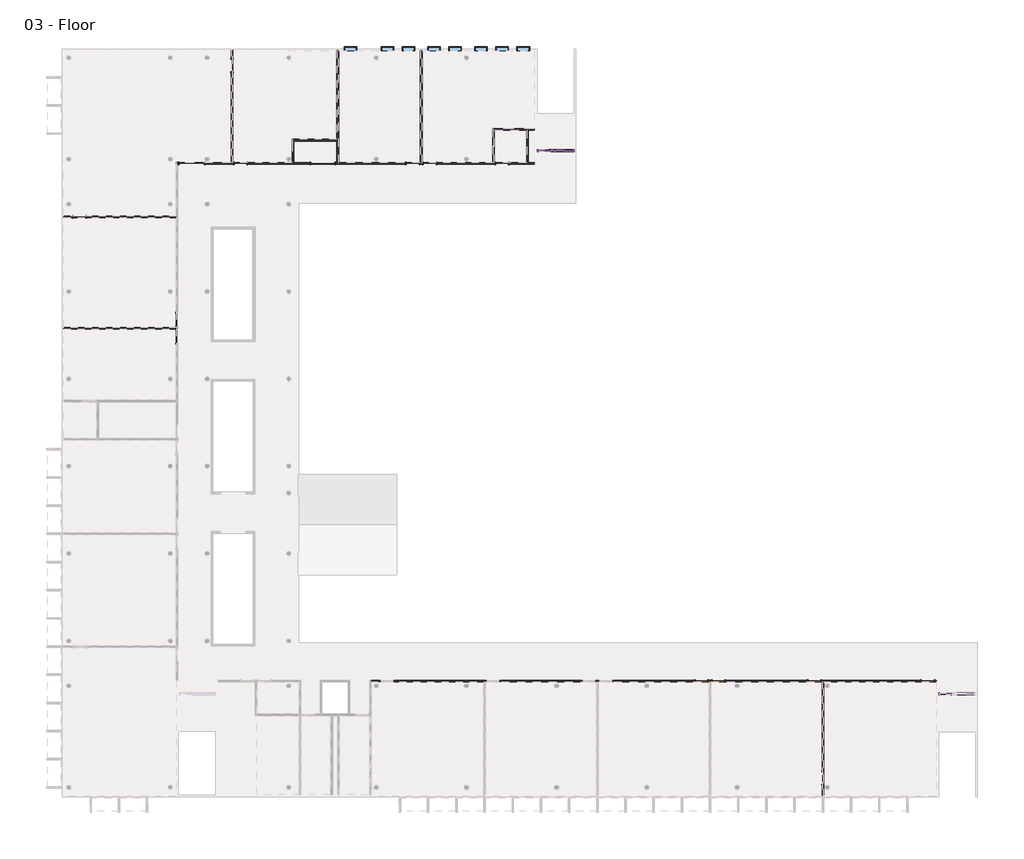
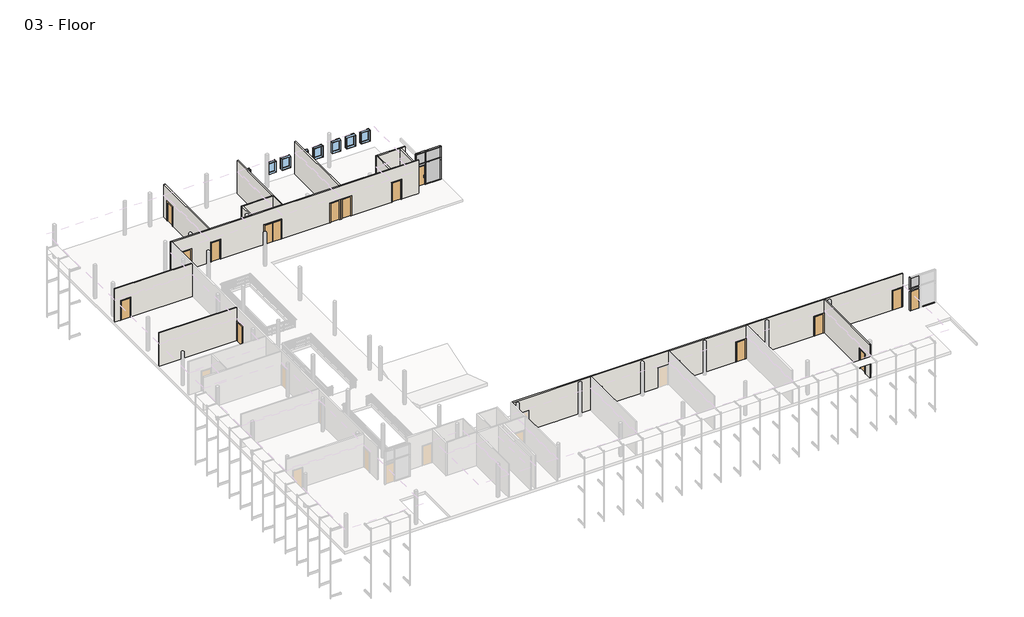
# One storey, part 2 of 4: 22 members, 17 doors, 13 walls, 8 windows, 6 plates.
"""IFC4 building model written with IfcOpenShell, lengths in millimetres."""

import ifcopenshell
import ifcopenshell.guid

model = None  # the IFC model being written
_history = None  # IfcOwnerHistory: only IFC2X3 demands one
_inside = {}  # id of a spatial element -> (the spatial element, [elements in it])
_under = {}  # id of a project, library or spatial element -> (it, [spatial elements below it])
_declared = {}  # id of a project -> (the project, [libraries it declares])
_typed = {}  # id of a type object -> (the type object, [elements of that type])
_made_of = {}  # id of a material, layer set ... -> (it, [elements and type objects made of it])


def new_model(schema):
    """Start an empty IFC model of exactly this schema.

    Asked for "IFC4X3", IfcOpenShell would pick the latest addendum, in which some entities
    have other attributes; the version numbers below select the first issue.
    IFC2X3 requires an IfcOwnerHistory on every rooted entity: one is made here for all.
    """
    global model, _history
    if schema == "IFC4X3":
        model = ifcopenshell.file(schema_version=(4, 3, 0, 0))
    else:
        model = ifcopenshell.file(schema=schema)
    _inside.clear()
    _under.clear()
    _declared.clear()
    _typed.clear()
    _made_of.clear()
    _history = None
    if model.schema == "IFC2X3":
        org = make("IfcOrganization", Name="unknown")
        user = make(
            "IfcPersonAndOrganization",
            ThePerson=make("IfcPerson", FamilyName="unknown"),
            TheOrganization=org,
        )
        app = make(
            "IfcApplication",
            ApplicationDeveloper=org,
            Version="unknown",
            ApplicationFullName="unknown",
            ApplicationIdentifier="unknown",
        )
        _history = make(
            "IfcOwnerHistory",
            OwningUser=user,
            OwningApplication=app,
            ChangeAction="ADDED",
            CreationDate=0,
        )
    return model


def make(cls, **values):
    """One entity of the class cls with the attributes given. An attribute that is None is left unset."""
    return model.create_entity(
        cls, **{name: value for name, value in values.items() if value is not None}
    )


def rooted(cls, **values):
    """An entity with a GlobalId (a new one), such as an element, a storey or a relation."""
    return make(cls, GlobalId=ifcopenshell.guid.new(), OwnerHistory=_history, **values)


def si_unit(unit_type, name, prefix=None):
    """IfcSIUnit, for example si_unit("LENGTHUNIT", "METRE", prefix="MILLI")."""
    return make("IfcSIUnit", UnitType=unit_type, Prefix=prefix, Name=name)


def assignment(units):
    """IfcUnitAssignment: the units of a project."""
    return None if units is None else make("IfcUnitAssignment", Units=units)


def point(xyz):
    """IfcCartesianPoint."""
    return None if xyz is None else make("IfcCartesianPoint", Coordinates=xyz)


def direction(xyz):
    """IfcDirection."""
    return None if xyz is None else make("IfcDirection", DirectionRatios=xyz)


def frame(location, z_axis=None, x_axis=None):
    """IfcAxis2Placement3D, a coordinate frame: its origin and axes. An axis left out is left unset."""
    return make(
        "IfcAxis2Placement3D",
        Location=point(location),
        Axis=direction(z_axis),
        RefDirection=direction(x_axis),
    )


def origin():
    """The frame at (0, 0, 0) with its axes left unset."""
    return frame((0.0, 0.0, 0.0))


def origin_with_axes():
    """The frame at (0, 0, 0) with the z axis (0, 0, 1) and the x axis (1, 0, 0) written out."""
    return frame((0.0, 0.0, 0.0), z_axis=(0.0, 0.0, 1.0), x_axis=(1.0, 0.0, 0.0))


def place(relative_to, where):
    """IfcLocalPlacement: puts the frame where relative to a parent placement (None: the world)."""
    return make(
        "IfcLocalPlacement", PlacementRelTo=relative_to, RelativePlacement=where
    )


def context(
    kind, dimensions, precision=None, world=None, true_north=None, identifier=None
):
    """IfcGeometricRepresentationContext, for example the 3D "Model" context."""
    return make(
        "IfcGeometricRepresentationContext",
        ContextIdentifier=identifier,
        ContextType=kind,
        CoordinateSpaceDimension=dimensions,
        Precision=precision,
        WorldCoordinateSystem=world,
        TrueNorth=true_north,
    )


def project(units=None, contexts=None):
    """IfcProject with its units and contexts."""
    return rooted(
        "IfcProject",
        Name="project",
        RepresentationContexts=contexts,
        UnitsInContext=assignment(units),
    )


def spatial(cls, under=None, at=None, **own):
    """A site, building, storey or space (cls), placed at a placement, below another one or the project."""
    s = rooted(cls, ObjectPlacement=at, **own)
    if under is not None:
        _under.setdefault(under.id(), (under, []))[1].append(s)
    return s


def polyline(points):
    """IfcPolyline through the points."""
    return make("IfcPolyline", Points=[point(p) for p in points])


def outline(outer, holes=None, kind="AREA"):
    """IfcArbitraryClosedProfileDef: a profile drawn as a closed curve; with holes, ...WithVoids."""
    if holes is None:
        return make("IfcArbitraryClosedProfileDef", ProfileType=kind, OuterCurve=outer)
    return make(
        "IfcArbitraryProfileDefWithVoids",
        ProfileType=kind,
        OuterCurve=outer,
        InnerCurves=holes,
    )


def extrude(swept, where, along, depth):
    """IfcExtrudedAreaSolid: the profile swept, set in the frame where, extruded along a direction by depth."""
    return make(
        "IfcExtrudedAreaSolid",
        SweptArea=swept,
        Position=where,
        ExtrudedDirection=direction(along),
        Depth=depth,
    )


def faces_of(points, faces, orient=None, outer=None):
    """IfcFace entities. A face is a list of loops; a loop is a list of indices into points, from 0.

    orient and outer hold one flag for each loop. By default every Orientation is true, the
    first loop of a face is its IfcFaceOuterBound and the others are IfcFaceBound.
    """
    made = []
    for i, loops in enumerate(faces):
        bounds = []
        for j, loop in enumerate(loops):
            is_outer = j == 0 if outer is None else outer[i][j]
            bounds.append(
                make(
                    "IfcFaceOuterBound" if is_outer else "IfcFaceBound",
                    Bound=make("IfcPolyLoop", Polygon=[points[k] for k in loop]),
                    Orientation=True if orient is None else orient[i][j],
                )
            )
        made.append(make("IfcFace", Bounds=bounds))
    return made


def faceted_brep(points, faces, orient=None, outer=None, voids=None):
    """IfcFacetedBrep: a solid bounded by flat faces; with voids (closed shells), ...WithVoids."""
    shared = [point(p) for p in points]
    hull = make("IfcClosedShell", CfsFaces=faces_of(shared, faces, orient, outer))
    if voids is None:
        return make("IfcFacetedBrep", Outer=hull)
    return make(
        "IfcFacetedBrepWithVoids",
        Outer=hull,
        Voids=[
            make(cls, CfsFaces=faces_of(shared, fs, o, b)) for cls, fs, o, b in voids
        ],
    )


def shape(context_of_items, identifier, shape_type, items):
    """IfcShapeRepresentation: the items that make up one representation, for example the "Body"."""
    return make(
        "IfcShapeRepresentation",
        ContextOfItems=context_of_items,
        RepresentationIdentifier=identifier,
        RepresentationType=shape_type,
        Items=items,
    )


def source(mapping_origin, context_of_items, identifier, shape_type, items):
    """IfcRepresentationMap: a shape defined once, which mapped items show again and again."""
    return make(
        "IfcRepresentationMap",
        MappingOrigin=mapping_origin,
        MappedRepresentation=shape(context_of_items, identifier, shape_type, items),
    )


def transform(
    local_origin,
    x_axis=None,
    y_axis=None,
    z_axis=None,
    scale=None,
    scale2=None,
    scale3=None,
    uniform=True,
):
    """IfcCartesianTransformationOperator3D, or its non-uniform kind. x_axis, y_axis, z_axis: its Axis1, 2, 3."""
    if uniform:
        return make(
            "IfcCartesianTransformationOperator3D",
            Axis1=direction(x_axis),
            Axis2=direction(y_axis),
            LocalOrigin=point(local_origin),
            Scale=scale,
            Axis3=direction(z_axis),
        )
    return make(
        "IfcCartesianTransformationOperator3DnonUniform",
        Axis1=direction(x_axis),
        Axis2=direction(y_axis),
        LocalOrigin=point(local_origin),
        Scale=scale,
        Axis3=direction(z_axis),
        Scale2=scale2,
        Scale3=scale3,
    )


def mapped(mapping_source, mapping_target):
    """IfcMappedItem: shows the shape of a source again, moved by a transform."""
    return make(
        "IfcMappedItem", MappingSource=mapping_source, MappingTarget=mapping_target
    )


def made_of(thing, what):
    """Note that an element or type object is made of a material, layer set ...; save() writes the relation."""
    if what is not None:
        _made_of.setdefault(what.id(), (what, []))[1].append(thing)
    return thing


def element(
    cls,
    number,
    at=None,
    inside=None,
    cuts=None,
    type_object=None,
    material=None,
    context=None,
    identifier="Body",
    shape_type=None,
    held_by="IfcProductDefinitionShape",
    body=None,
    shapes=None,
    **own,
):
    """One element of the class cls, such as IfcWall. Its Tag is "e" and its number.

    at: its placement. inside: the storey or other place that contains it. cuts: it is an
    opening in that element (IfcRelVoidsElement). A single representation is given by context,
    identifier, shape_type and body (its items); several are given by shapes. held_by: the class
    of the entity that holds the representations. save() writes the other relations.
    """
    e = rooted(cls, Tag="e%d" % number, ObjectPlacement=at, **own)
    if body is not None:
        shapes = [shape(context, identifier, shape_type, body)]
    if shapes is not None:
        e.Representation = make(held_by, Representations=shapes)
    if inside is not None:
        _inside.setdefault(inside.id(), (inside, []))[1].append(e)
    if cuts is not None:
        rooted(
            "IfcRelVoidsElement", RelatingBuildingElement=cuts, RelatedOpeningElement=e
        )
    if type_object is not None:
        _typed.setdefault(type_object.id(), (type_object, []))[1].append(e)
    return made_of(e, material)


def aggregate(whole, parts):
    """IfcRelAggregates: a whole, such as a stair, and the parts it consists of."""
    return rooted("IfcRelAggregates", RelatingObject=whole, RelatedObjects=parts)


def save(model, path):
    """Write the relations noted so far, then the file.

    IfcRelAggregates (storeys below a building ...), IfcRelContainedInSpatialStructure (elements
    in a storey), IfcRelDefinesByType, IfcRelAssociatesMaterial and IfcRelDeclares: one each for
    every whole, place, type object, material and project.
    """
    for whole, parts in _under.values():
        aggregate(whole, parts)
    for where, things in _inside.values():
        rooted(
            "IfcRelContainedInSpatialStructure",
            RelatedElements=things,
            RelatingStructure=where,
        )
    for kind, things in _typed.values():
        rooted("IfcRelDefinesByType", RelatedObjects=things, RelatingType=kind)
    for what, things in _made_of.values():
        rooted("IfcRelAssociatesMaterial", RelatedObjects=things, RelatingMaterial=what)
    for by, libraries in _declared.values():
        rooted("IfcRelDeclares", RelatingContext=by, RelatedDefinitions=libraries)
    model.write(path)


def curtain_wall_sgl_glass_curtain_wall_sgl_glass_c2d4b377(model_context):
    return source(origin(), model_context, "Body", "SweptSolid", [
        extrude(outline(polyline([(-355.6, 12.7), (-355.6, -38.1), (-381.0, -38.1), (-381.0, 12.7), (-355.6, 12.7)])), frame((0.0, 0.0, 762.0), z_axis=(0.0, 0.0, 1.0), x_axis=(1.0, 0.0, 0.0)), (0.0, 0.0, 1.0), 228.6),
        extrude(outline(polyline([(-381.0, -101.6), (-381.0, -50.8), (-355.6, -50.8), (-355.6, -101.6), (-381.0, -101.6)])), frame((0.0, 0.0, 762.0), z_axis=(0.0, 0.0, 1.0), x_axis=(1.0, 0.0, 0.0)), (0.0, 0.0, 1.0), 228.6),
        extrude(outline(polyline([(457.2, -50.8), (-457.2, -50.8), (-457.2, -38.1), (457.2, -38.1), (457.2, -50.8)])), origin_with_axes(), (0.0, 0.0, 1.0), 2133.6),
    ])


def curtain_wall_sgl_glass_curtain_wall_sgl_glass_ab2568d1(model_context):
    return source(origin(), model_context, "Body", "SweptSolid", [
        extrude(outline(polyline([(-355.6, -12.7), (-381.0, -12.7), (-381.0, 38.1), (-355.6, 38.1), (-355.6, -12.7)])), frame((0.0, 0.0, 762.0), z_axis=(0.0, 0.0, 1.0), x_axis=(1.0, 0.0, 0.0)), (0.0, 0.0, 1.0), 228.6),
        extrude(outline(polyline([(-381.0, 101.6), (-355.6, 101.6), (-355.6, 50.8), (-381.0, 50.8), (-381.0, 101.6)])), frame((0.0, 0.0, 762.0), z_axis=(0.0, 0.0, 1.0), x_axis=(1.0, 0.0, 0.0)), (0.0, 0.0, 1.0), 228.6),
        extrude(outline(polyline([(457.2, 50.8), (457.2, 38.1), (-457.2, 38.1), (-457.2, 50.8), (457.2, 50.8)])), origin_with_axes(), (0.0, 0.0, 1.0), 2133.6),
    ])


def door_63ee19b0(model_context):
    return source(origin(), model_context, "Body", "SweptSolid", [
        extrude(outline(polyline([(0.0, -57.15), (0.0, -6.35), (863.6, -6.35), (863.6, -57.15), (0.0, -57.15)])), origin_with_axes(), (0.0, 0.0, 1.0), 2133.6),
        extrude(outline(polyline([(-863.6, -57.15), (-863.6, -6.35), (0.0, -6.35), (0.0, -57.15), (-863.6, -57.15)])), origin_with_axes(), (0.0, 0.0, 1.0), 2133.6),
        extrude(outline(polyline([(2133.6, -863.6), (2133.6, 863.6), (0.0, 863.6), (0.0, 939.8), (2209.8, 939.8), (2209.8, -939.8), (0.0, -939.8), (0.0, -863.6), (2133.6, -863.6)])), frame((0.0, 57.15, 0.0), z_axis=(0.0, 1.0, 0.0), x_axis=(0.0, 0.0, 1.0)), (0.0, 0.0, 1.0), 25.4),
        extrude(outline(polyline([(2133.6, -863.6), (2133.6, 863.6), (0.0, 863.6), (0.0, 939.8), (2209.8, 939.8), (2209.8, -939.8), (0.0, -939.8), (0.0, -863.6), (2133.6, -863.6)])), frame((0.0, -82.55, 0.0), z_axis=(0.0, 1.0, 0.0), x_axis=(0.0, 0.0, 1.0)), (0.0, 0.0, 1.0), 25.4),
    ])


def door_3e29e47a(model_context):
    return source(origin(), model_context, "Body", "SweptSolid", [
        extrude(outline(polyline([(0.0, 57.15), (914.4, 57.15), (914.4, 6.35), (0.0, 6.35), (0.0, 57.15)])), origin_with_axes(), (0.0, 0.0, 1.0), 2133.6),
        extrude(outline(polyline([(-914.4, 57.15), (0.0, 57.15), (0.0, 6.35), (-914.4, 6.35), (-914.4, 57.15)])), origin_with_axes(), (0.0, 0.0, 1.0), 2133.6),
        extrude(outline(polyline([(2133.6, -914.4), (2133.6, 914.4), (0.0, 914.4), (0.0, 990.6), (2209.8, 990.6), (2209.8, -990.6), (0.0, -990.6), (0.0, -914.4), (2133.6, -914.4)])), frame((0.0, -82.55, 0.0), z_axis=(0.0, 1.0, 0.0), x_axis=(0.0, 0.0, 1.0)), (0.0, 0.0, 1.0), 25.4),
        extrude(outline(polyline([(2133.6, -914.4), (2133.6, 914.4), (0.0, 914.4), (0.0, 990.6), (2209.8, 990.6), (2209.8, -990.6), (0.0, -990.6), (0.0, -914.4), (2133.6, -914.4)])), frame((0.0, 57.15, 0.0), z_axis=(0.0, 1.0, 0.0), x_axis=(0.0, 0.0, 1.0)), (0.0, 0.0, 1.0), 25.4),
    ])


def door_305aa2a5(model_context):
    return source(origin(), model_context, "Body", "SweptSolid", [
        extrude(outline(polyline([(2209.8, -533.4), (0.0, -533.4), (0.0, -457.2), (2133.6, -457.2), (2133.6, 457.2), (0.0, 457.2), (0.0, 533.4), (2209.8, 533.4), (2209.8, -533.4)])), frame((0.0, -82.55, 0.0), z_axis=(0.0, 1.0, 0.0), x_axis=(0.0, 0.0, 1.0)), (0.0, 0.0, 1.0), 25.4),
        extrude(outline(polyline([(2209.8, 533.4), (2209.8, -533.4), (0.0, -533.4), (0.0, -457.2), (2133.6, -457.2), (2133.6, 457.2), (0.0, 457.2), (0.0, 533.4), (2209.8, 533.4)])), frame((0.0, 57.15, 0.0), z_axis=(0.0, 1.0, 0.0), x_axis=(0.0, 0.0, 1.0)), (0.0, 0.0, 1.0), 25.4),
        extrude(outline(polyline([(457.2, -6.35), (457.2, -57.15), (-457.2, -57.15), (-457.2, -6.35), (457.2, -6.35)])), origin_with_axes(), (0.0, 0.0, 1.0), 2133.6),
    ])


def door_e5f9f3c4(model_context):
    return source(origin(), model_context, "Body", "SweptSolid", [
        extrude(outline(polyline([(2209.8, -533.4), (0.0, -533.4), (0.0, -457.2), (2133.6, -457.2), (2133.6, 457.2), (0.0, 457.2), (0.0, 533.4), (2209.8, 533.4), (2209.8, -533.4)])), frame((0.0, 57.15, 0.0), z_axis=(0.0, 1.0, 0.0), x_axis=(0.0, 0.0, 1.0)), (0.0, 0.0, 1.0), 25.4),
        extrude(outline(polyline([(2209.8, 533.4), (2209.8, -533.4), (0.0, -533.4), (0.0, -457.2), (2133.6, -457.2), (2133.6, 457.2), (0.0, 457.2), (0.0, 533.4), (2209.8, 533.4)])), frame((0.0, -82.55, 0.0), z_axis=(0.0, 1.0, 0.0), x_axis=(0.0, 0.0, 1.0)), (0.0, 0.0, 1.0), 25.4),
        extrude(outline(polyline([(457.2, 6.35), (-457.2, 6.35), (-457.2, 57.15), (457.2, 57.15), (457.2, 6.35)])), origin_with_axes(), (0.0, 0.0, 1.0), 2133.6),
    ])


def member_2b49869a(model_context):
    return source(origin(), model_context, "Body", "SweptSolid", [
        extrude(outline(polyline([(31.75, 63.5), (31.75, -63.5), (-31.75, -63.5), (-31.75, 63.5), (31.75, 63.5)])), frame((0.0, 0.0, -1219.2), z_axis=(0.0, 0.0, 1.0), x_axis=(1.0, 0.0, 0.0)), (0.0, 0.0, 1.0), 1219.2),
    ])


def member_75074519(model_context):
    return source(origin(), model_context, "Body", "SweptSolid", [
        extrude(outline(polyline([(0.0, 63.5), (0.0, -63.5), (-63.5, -63.5), (-63.5, 63.5), (0.0, 63.5)])), frame((0.0, 0.0, -1219.2), z_axis=(0.0, 0.0, 1.0), x_axis=(1.0, 0.0, 0.0)), (0.0, 0.0, 1.0), 1219.2),
    ])


def member_6186cc23(model_context):
    return source(origin(), model_context, "Body", "SweptSolid", [
        extrude(outline(polyline([(31.75, 63.5), (31.75, -63.5), (-31.75, -63.5), (-31.75, 63.5), (31.75, 63.5)])), frame((0.0, 0.0, -2165.35), z_axis=(0.0, 0.0, 1.0), x_axis=(1.0, 0.0, 0.0)), (0.0, 0.0, 1.0), 2165.35),
    ])


def member_5d67b9fc(model_context):
    return source(origin(), model_context, "Body", "SweptSolid", [
        extrude(outline(polyline([(31.75, 63.5), (31.75, -63.5), (-31.75, -63.5), (-31.75, 63.5), (31.75, 63.5)])), frame((0.0, 0.0, -273.05), z_axis=(0.0, 0.0, 1.0), x_axis=(1.0, 0.0, 0.0)), (0.0, 0.0, 1.0), 273.05),
    ])


def member_a50b3cda(model_context):
    return source(origin(), model_context, "Body", "SweptSolid", [
        extrude(outline(polyline([(0.0, 63.5), (0.0, -63.5), (-63.5, -63.5), (-63.5, 63.5), (0.0, 63.5)])), frame((0.0, 0.0, -2165.35), z_axis=(0.0, 0.0, 1.0), x_axis=(1.0, 0.0, 0.0)), (0.0, 0.0, 1.0), 2165.35),
    ])


def member_c327c56d(model_context):
    return source(origin(), model_context, "Body", "SweptSolid", [
        extrude(outline(polyline([(0.0, 63.5), (0.0, -63.5), (-63.5, -63.5), (-63.5, 63.5), (0.0, 63.5)])), frame((0.0, 0.0, -273.05), z_axis=(0.0, 0.0, 1.0), x_axis=(1.0, 0.0, 0.0)), (0.0, 0.0, 1.0), 273.05),
    ])


def member_410c6227(model_context):
    return source(origin(), model_context, "Body", "SweptSolid", [
        extrude(outline(polyline([(31.75, 63.5), (31.75, -63.5), (-31.75, -63.5), (-31.75, 63.5), (31.75, 63.5)])), frame((0.0, 0.0, -914.4), z_axis=(0.0, 0.0, 1.0), x_axis=(1.0, 0.0, 0.0)), (0.0, 0.0, 1.0), 914.4),
    ])


def member_73c23c35(model_context):
    return source(origin(), model_context, "Body", "SweptSolid", [
        extrude(outline(polyline([(0.0, 63.5), (0.0, -63.5), (-63.5, -63.5), (-63.5, 63.5), (0.0, 63.5)])), frame((0.0, 0.0, -914.4), z_axis=(0.0, 0.0, 1.0), x_axis=(1.0, 0.0, 0.0)), (0.0, 0.0, 1.0), 914.4),
    ])


def member_bcb6a316(model_context):
    return source(origin(), model_context, "Body", "SweptSolid", [
        extrude(outline(polyline([(0.0, 63.5), (0.0, -63.5), (-63.5, -63.5), (-63.5, 63.5), (0.0, 63.5)])), frame((0.0, 0.0, -1257.3), z_axis=(0.0, 0.0, 1.0), x_axis=(1.0, 0.0, 0.0)), (0.0, 0.0, 1.0), 1257.3),
    ])


def member_d3323a85(model_context):
    return source(origin(), model_context, "Body", "SweptSolid", [
        extrude(outline(polyline([(0.0, 63.5), (0.0, -63.5), (-63.5, -63.5), (-63.5, 63.5), (0.0, 63.5)])), frame((0.0, 0.0, -279.4), z_axis=(0.0, 0.0, 1.0), x_axis=(1.0, 0.0, 0.0)), (0.0, 0.0, 1.0), 279.4),
    ])


def member_7bd2cd2c(model_context):
    return source(origin(), model_context, "Body", "SweptSolid", [
        extrude(outline(polyline([(31.75, 63.5), (31.75, -63.5), (-31.75, -63.5), (-31.75, 63.5), (31.75, 63.5)])), frame((0.0, 0.0, -1257.3), z_axis=(0.0, 0.0, 1.0), x_axis=(1.0, 0.0, 0.0)), (0.0, 0.0, 1.0), 1257.3),
    ])


def member_6be37683(model_context):
    return source(origin(), model_context, "Body", "SweptSolid", [
        extrude(outline(polyline([(31.75, 63.5), (31.75, -63.5), (-31.75, -63.5), (-31.75, 63.5), (31.75, 63.5)])), frame((0.0, 0.0, -279.4), z_axis=(0.0, 0.0, 1.0), x_axis=(1.0, 0.0, 0.0)), (0.0, 0.0, 1.0), 279.4),
    ])


def member_e7b2e991(model_context):
    return source(origin(), model_context, "Body", "SweptSolid", [
        extrude(outline(polyline([(0.0, 63.5), (0.0, -63.5), (-63.5, -63.5), (-63.5, 63.5), (0.0, 63.5)])), frame((0.0, 0.0, -1263.65), z_axis=(0.0, 0.0, 1.0), x_axis=(1.0, 0.0, 0.0)), (0.0, 0.0, 1.0), 1263.65),
    ])


def system_panel_glazed_8dc8626f(model_context):
    return source(origin(), model_context, "Body", "SweptSolid", [
        extrude(outline(polyline([(457.2, -44.45), (-457.2, -44.45), (-457.2, -19.05), (457.2, -19.05), (457.2, -44.45)])), origin_with_axes(), (0.0, 0.0, 1.0), 209.55),
    ])


def system_panel_glazed_bb2f95a6(model_context):
    return source(origin(), model_context, "Body", "SweptSolid", [
        extrude(outline(polyline([(0.0, -768.35), (0.0, -488.95), (0.0, 768.35), (2101.85, 768.35), (2343.15, 768.35), (2343.15, -488.95), (2343.15, -768.35), (2101.85, -768.35), (0.0, -768.35)])), frame((0.0, -44.45, 0.0), z_axis=(0.0, 1.0, 0.0), x_axis=(0.0, 0.0, 1.0)), (0.0, 0.0, 1.0), 25.4),
    ])


def system_panel_glazed_2e5f6ce9(model_context):
    return source(origin(), model_context, "Body", "SweptSolid", [
        extrude(outline(polyline([(457.2, -44.45), (-457.2, -44.45), (-457.2, -19.05), (457.2, -19.05), (457.2, -44.45)])), origin_with_axes(), (0.0, 0.0, 1.0), 1123.95),
    ])


def system_panel_glazed_639f3d85(model_context):
    return source(origin(), model_context, "Body", "SweptSolid", [
        extrude(outline(polyline([(0.0, -768.35), (0.0, -488.95), (0.0, 768.35), (1123.95, 768.35), (1123.95, -488.95), (1123.95, -768.35), (0.0, -768.35)])), frame((0.0, -44.45, 0.0), z_axis=(0.0, 1.0, 0.0), x_axis=(0.0, 0.0, 1.0)), (0.0, 0.0, 1.0), 25.4),
    ])


def system_panel_glazed_72fe8651(model_context):
    return source(origin(), model_context, "Body", "SweptSolid", [
        extrude(outline(polyline([(457.2, 19.05), (-457.2, 19.05), (-457.2, 44.45), (457.2, 44.45), (457.2, 19.05)])), origin_with_axes(), (0.0, 0.0, 1.0), 209.55),
    ])


def system_panel_glazed_1925881f(model_context):
    return source(origin(), model_context, "Body", "SweptSolid", [
        extrude(outline(polyline([(457.2, 19.05), (-457.2, 19.05), (-457.2, 44.45), (457.2, 44.45), (457.2, 19.05)])), origin_with_axes(), (0.0, 0.0, 1.0), 1123.95),
    ])


def window_dfee3f32(model_context):
    return source(origin(), model_context, "Body", "SweptSolid", [
        extrude(outline(polyline([(355.6, 106.3625), (-431.8, 106.3625), (-431.8, 119.0625), (355.6, 119.0625), (355.6, 106.3625)])), frame((0.0, 0.0, 977.9), z_axis=(0.0, 0.0, 1.0), x_axis=(1.0, 0.0, 0.0)), (0.0, 0.0, 1.0), 1092.2),
        extrude(outline(polyline([(2114.55, -476.25), (933.45, -476.25), (933.45, 400.05), (2114.55, 400.05), (2114.55, -476.25)]), holes=[polyline([(2070.1, -431.8), (2070.1, 355.6), (977.9, 355.6), (977.9, -431.8), (2070.1, -431.8)])]), frame((0.0, 90.4875, 0.0), z_axis=(0.0, 1.0, 0.0), x_axis=(0.0, 0.0, 1.0)), (0.0, 0.0, 1.0), 44.45),
        extrude(outline(polyline([(2133.6, -495.3), (914.4, -495.3), (914.4, 419.1), (2133.6, 419.1), (2133.6, -495.3)]), holes=[polyline([(2101.85, -463.55), (2101.85, 387.35), (946.15, 387.35), (946.15, -463.55), (2101.85, -463.55)])]), frame((0.0, -153.9875, 0.0), z_axis=(0.0, 1.0, 0.0), x_axis=(0.0, 0.0, 1.0)), (0.0, 0.0, 1.0), 244.475),
        extrude(outline(polyline([(2133.6, 419.1), (2133.6, -495.3), (914.4, -495.3), (914.4, 419.1), (2133.6, 419.1)]), holes=[polyline([(2114.55, 400.05), (933.45, 400.05), (933.45, -476.25), (2114.55, -476.25), (2114.55, 400.05)])]), frame((0.0, 90.4875, 0.0), z_axis=(0.0, 1.0, 0.0), x_axis=(0.0, 0.0, 1.0)), (0.0, 0.0, 1.0), 63.5),
    ])


model = new_model("IFC4")

# Units and contexts
model_context = context("Model", 3, world=origin())
ifc_project = project(units=[si_unit("LENGTHUNIT", "METRE", prefix="MILLI")], contexts=[model_context])

# Site, building, storey
site = spatial("IfcSite", under=ifc_project)
building = spatial("IfcBuilding", under=site)
storey = spatial("IfcBuildingStorey", under=building, Name="03 - Floor", Elevation=7315.2)

# Doors
placement = place(None, origin())
curtain_wall_sgl_glass_curtain_wall_sgl_glass_shape = curtain_wall_sgl_glass_curtain_wall_sgl_glass_c2d4b377(model_context)
element("IfcDoor", 1, ObjectType="Curtain Wall Sgl Glass : Curtain Wall Sgl Glass", at=placement, inside=storey, context=model_context, shape_type="MappedRepresentation", body=[
    mapped(curtain_wall_sgl_glass_curtain_wall_sgl_glass_shape, transform((34925.9207476, 46523.2, 7315.2), x_axis=(-1.0, 0.0, 0.0), y_axis=(0.0, -1.0, 0.0), z_axis=(0.0, 0.0, 1.0))),
])
curtain_wall_sgl_glass_curtain_wall_sgl_glass_2_shape = curtain_wall_sgl_glass_curtain_wall_sgl_glass_ab2568d1(model_context)
element("IfcDoor", 2, ObjectType="Curtain Wall Sgl Glass : Curtain Wall Sgl Glass", at=placement, inside=storey, context=model_context, shape_type="MappedRepresentation", body=[
    mapped(curtain_wall_sgl_glass_curtain_wall_sgl_glass_2_shape, transform((63869.2207476, 7356.4, 7315.2), x_axis=(-1.0, 0.0, 0.0), y_axis=(0.0, -1.0, 0.0), z_axis=(0.0, 0.0, 1.0))),
])
door_shape = door_63ee19b0(model_context)
element("IfcDoor", 3, ObjectType="Double-Flush : 68\" x 84\"", at=placement, inside=storey, context=model_context, shape_type="MappedRepresentation", body=[
    mapped(door_shape, transform((18949.3207476, 45602.45, 7315.2), x_axis=(1.0, 0.0, 0.0), y_axis=(0.0, 1.0, 0.0), z_axis=(0.0, 0.0, 1.0))),
])
door_2_shape = door_3e29e47a(model_context)
element("IfcDoor", 4, ObjectType="Double-Flush : 72\" x 84\"", at=placement, inside=storey, context=model_context, shape_type="MappedRepresentation", body=[
    mapped(door_2_shape, transform((9487.8207476, 45602.45, 7315.2), x_axis=(1.0, 0.0, 0.0), y_axis=(0.0, 1.0, 0.0), z_axis=(0.0, 0.0, 1.0))),
])
door_3_shape = door_305aa2a5(model_context)
element("IfcDoor", 5, ObjectType="Single-Flush : 36\" x 84\"", at=placement, inside=storey, context=model_context, shape_type="MappedRepresentation", body=[
    mapped(door_3_shape, transform((31865.2207476, 45602.45, 7315.2), x_axis=(-1.0, 0.0, 0.0), y_axis=(0.0, -1.0, 0.0), z_axis=(0.0, 0.0, 1.0))),
])
element("IfcDoor", 6, ObjectType="Single-Flush : 36\" x 84\"", at=placement, inside=storey, context=model_context, shape_type="MappedRepresentation", body=[
    mapped(door_3_shape, transform((26645.5207476, 45602.45, 7315.2), x_axis=(-1.0, 0.0, 0.0), y_axis=(0.0, -1.0, 0.0), z_axis=(0.0, 0.0, 1.0))),
])
element("IfcDoor", 7, ObjectType="Single-Flush : 36\" x 84\"", at=placement, inside=storey, context=model_context, shape_type="MappedRepresentation", body=[
    mapped(door_3_shape, transform((13005.7207476, 45602.45, 7315.2), x_axis=(-1.0, 0.0, 0.0), y_axis=(0.0, -1.0, 0.0), z_axis=(0.0, 0.0, 1.0))),
])
element("IfcDoor", 8, ObjectType="Single-Flush : 36\" x 84\"", at=placement, inside=storey, context=model_context, shape_type="MappedRepresentation", body=[
    mapped(door_3_shape, transform((8414.6707476, 34331.2, 7315.2), x_axis=(0.0, -1.0, 0.0), y_axis=(1.0, 0.0, 0.0), z_axis=(0.0, 0.0, 1.0))),
])
element("IfcDoor", 9, ObjectType="Single-Flush : 36\" x 84\"", at=placement, inside=storey, context=model_context, shape_type="MappedRepresentation", body=[
    mapped(door_3_shape, transform((12396.1207476, 52657.3, 7315.2), x_axis=(0.0, 1.0, 0.0), y_axis=(-1.0, 0.0, 0.0), z_axis=(0.0, 0.0, 1.0))),
])
element("IfcDoor", 10, ObjectType="Single-Flush : 36\" x 84\"", at=placement, inside=storey, context=model_context, shape_type="MappedRepresentation", body=[
    mapped(door_3_shape, transform((46241.6207476, 8277.15, 7315.2), x_axis=(1.0, 0.0, 0.0), y_axis=(0.0, 1.0, 0.0), z_axis=(0.0, 0.0, 1.0))),
])
element("IfcDoor", 11, ObjectType="Single-Flush : 36\" x 84\"", at=placement, inside=storey, context=model_context, shape_type="MappedRepresentation", body=[
    mapped(door_3_shape, transform((54369.6207476, 8277.15, 7315.2), x_axis=(1.0, 0.0, 0.0), y_axis=(0.0, 1.0, 0.0), z_axis=(0.0, 0.0, 1.0))),
])
element("IfcDoor", 12, ObjectType="Single-Flush : 36\" x 84\"", at=placement, inside=storey, context=model_context, shape_type="MappedRepresentation", body=[
    mapped(door_3_shape, transform((62535.7207476, 8277.15, 7315.2), x_axis=(1.0, 0.0, 0.0), y_axis=(0.0, 1.0, 0.0), z_axis=(0.0, 0.0, 1.0))),
])
door_4_shape = door_e5f9f3c4(model_context)
element("IfcDoor", 13, ObjectType="Single-Flush : 36\" x 84\"", at=placement, inside=storey, context=model_context, shape_type="MappedRepresentation", body=[
    mapped(door_4_shape, transform((25426.3207476, 45602.45, 7315.2), x_axis=(1.0, 0.0, 0.0), y_axis=(0.0, 1.0, 0.0), z_axis=(0.0, 0.0, 1.0))),
])
element("IfcDoor", 14, ObjectType="Single-Flush : 36\" x 84\"", at=placement, inside=storey, context=model_context, shape_type="MappedRepresentation", body=[
    mapped(door_4_shape, transform((1397.9207476, 41748.0, 7315.2), x_axis=(-1.0, 0.0, 0.0), y_axis=(0.0, -1.0, 0.0), z_axis=(0.0, 0.0, 1.0))),
])
element("IfcDoor", 15, ObjectType="Single-Flush : 36\" x 84\"", at=placement, inside=storey, context=model_context, shape_type="MappedRepresentation", body=[
    mapped(door_4_shape, transform((8414.6707476, 33112.0, 7315.2), x_axis=(0.0, 1.0, 0.0), y_axis=(-1.0, 0.0, 0.0), z_axis=(0.0, 0.0, 1.0))),
])
element("IfcDoor", 16, ObjectType="Single-Flush : 36\" x 84\"", at=placement, inside=storey, context=model_context, shape_type="MappedRepresentation", body=[
    mapped(door_4_shape, transform((47460.8207476, 8277.15, 7315.2), x_axis=(-1.0, 0.0, 0.0), y_axis=(0.0, -1.0, 0.0), z_axis=(0.0, 0.0, 1.0))),
])
element("IfcDoor", 17, ObjectType="Single-Flush : 36\" x 84\"", at=placement, inside=storey, context=model_context, shape_type="MappedRepresentation", body=[
    mapped(door_4_shape, transform((54979.2207476, 1273.1, 7315.2), x_axis=(0.0, -1.0, 0.0), y_axis=(1.0, 0.0, 0.0), z_axis=(0.0, 0.0, 1.0))),
])

# Members
member_shape = member_2b49869a(model_context)
element("IfcMember", 18, ObjectType="Rectangular Mullion : 2.5\" x 5\" rectangular", at=placement, inside=storey, context=model_context, shape_type="MappedRepresentation", body=[
    mapped(member_shape, transform((35414.8707476, 46523.2, 9753.6), x_axis=(1.0, 0.0, 0.0), y_axis=(0.0, -1.0, 0.0), z_axis=(0.0, 0.0, -1.0))),
])
member_2_shape = member_75074519(model_context)
element("IfcMember", 19, ObjectType="Rectangular Mullion : 2.5\" x 5\" rectangular", at=placement, inside=storey, context=model_context, shape_type="MappedRepresentation", body=[
    mapped(member_2_shape, transform((34405.2207476, 46523.2, 10972.8), x_axis=(-1.0, 0.0, 0.0), y_axis=(0.0, -1.0, 0.0), z_axis=(0.0, 0.0, 1.0))),
])
element("IfcMember", 20, ObjectType="Rectangular Mullion : 2.5\" x 5\" rectangular", at=placement, inside=storey, context=model_context, shape_type="MappedRepresentation", body=[
    mapped(member_2_shape, transform((37046.8207476, 46523.2, 9753.6), x_axis=(1.0, 0.0, 0.0), y_axis=(0.0, -1.0, 0.0), z_axis=(0.0, 0.0, -1.0))),
])
element("IfcMember", 21, ObjectType="Rectangular Mullion : 2.5\" x 5\" rectangular", at=placement, inside=storey, context=model_context, shape_type="MappedRepresentation", body=[
    mapped(member_2_shape, transform((63348.5207476, 7356.4, 10972.8), x_axis=(-1.0, 0.0, 0.0), y_axis=(0.0, -1.0, 0.0), z_axis=(0.0, 0.0, 1.0))),
])
member_3_shape = member_6186cc23(model_context)
element("IfcMember", 22, ObjectType="Rectangular Mullion : 2.5\" x 5\" rectangular", at=placement, inside=storey, context=model_context, shape_type="MappedRepresentation", body=[
    mapped(member_3_shape, transform((35414.8707476, 46523.2, 7315.2), x_axis=(1.0, 0.0, 0.0), y_axis=(0.0, -1.0, 0.0), z_axis=(0.0, 0.0, -1.0))),
])
member_4_shape = member_5d67b9fc(model_context)
element("IfcMember", 23, ObjectType="Rectangular Mullion : 2.5\" x 5\" rectangular", at=placement, inside=storey, context=model_context, shape_type="MappedRepresentation", body=[
    mapped(member_4_shape, transform((35414.8707476, 46523.2, 9480.55), x_axis=(1.0, 0.0, 0.0), y_axis=(0.0, -1.0, 0.0), z_axis=(0.0, 0.0, -1.0))),
])
member_5_shape = member_a50b3cda(model_context)
element("IfcMember", 24, ObjectType="Rectangular Mullion : 2.5\" x 5\" rectangular", at=placement, inside=storey, context=model_context, shape_type="MappedRepresentation", body=[
    mapped(member_5_shape, transform((37046.8207476, 46523.2, 7315.2), x_axis=(1.0, 0.0, 0.0), y_axis=(0.0, -1.0, 0.0), z_axis=(0.0, 0.0, -1.0))),
])
member_6_shape = member_c327c56d(model_context)
element("IfcMember", 25, ObjectType="Rectangular Mullion : 2.5\" x 5\" rectangular", at=placement, inside=storey, context=model_context, shape_type="MappedRepresentation", body=[
    mapped(member_6_shape, transform((37046.8207476, 46523.2, 9480.55), x_axis=(1.0, 0.0, 0.0), y_axis=(0.0, -1.0, 0.0), z_axis=(0.0, 0.0, -1.0))),
])
member_7_shape = member_410c6227(model_context)
element("IfcMember", 26, ObjectType="Rectangular Mullion : 2.5\" x 5\" rectangular", at=placement, inside=storey, context=model_context, shape_type="MappedRepresentation", body=[
    mapped(member_7_shape, transform((35383.1207476, 46523.2, 9753.6), x_axis=(0.0, 0.0, 1.0), y_axis=(0.0, -1.0, 0.0), z_axis=(1.0, 0.0, 0.0))),
])
element("IfcMember", 27, ObjectType="Rectangular Mullion : 2.5\" x 5\" rectangular", at=placement, inside=storey, context=model_context, shape_type="MappedRepresentation", body=[
    mapped(member_7_shape, transform((35383.1207476, 46523.2, 9480.55), x_axis=(0.0, 0.0, 1.0), y_axis=(0.0, -1.0, 0.0), z_axis=(1.0, 0.0, 0.0))),
])
member_8_shape = member_73c23c35(model_context)
element("IfcMember", 28, ObjectType="Rectangular Mullion : 2.5\" x 5\" rectangular", at=placement, inside=storey, context=model_context, shape_type="MappedRepresentation", body=[
    mapped(member_8_shape, transform((35383.1207476, 46523.2, 10972.8), x_axis=(0.0, 0.0, 1.0), y_axis=(0.0, -1.0, 0.0), z_axis=(1.0, 0.0, 0.0))),
])
element("IfcMember", 29, ObjectType="Rectangular Mullion : 2.5\" x 5\" rectangular", at=placement, inside=storey, context=model_context, shape_type="MappedRepresentation", body=[
    mapped(member_6_shape, transform((34405.2207476, 46523.2, 9753.6), x_axis=(-1.0, 0.0, 0.0), y_axis=(0.0, -1.0, 0.0), z_axis=(0.0, 0.0, 1.0))),
])
element("IfcMember", 30, ObjectType="Rectangular Mullion : 2.5\" x 5\" rectangular", at=placement, inside=storey, context=model_context, shape_type="MappedRepresentation", body=[
    mapped(member_5_shape, transform((34405.2207476, 46523.2, 9480.55), x_axis=(-1.0, 0.0, 0.0), y_axis=(0.0, -1.0, 0.0), z_axis=(0.0, 0.0, 1.0))),
])
member_9_shape = member_bcb6a316(model_context)
element("IfcMember", 31, ObjectType="Rectangular Mullion : 2.5\" x 5\" rectangular", at=placement, inside=storey, context=model_context, shape_type="MappedRepresentation", body=[
    mapped(member_9_shape, transform((35726.0207476, 46523.2, 7315.2), x_axis=(0.0, 0.0, -1.0), y_axis=(0.0, -1.0, 0.0), z_axis=(-1.0, 0.0, 0.0))),
])
member_10_shape = member_d3323a85(model_context)
element("IfcMember", 32, ObjectType="Rectangular Mullion : 2.5\" x 5\" rectangular", at=placement, inside=storey, context=model_context, shape_type="MappedRepresentation", body=[
    mapped(member_10_shape, transform((35446.6207476, 46523.2, 7315.2), x_axis=(0.0, 0.0, -1.0), y_axis=(0.0, -1.0, 0.0), z_axis=(-1.0, 0.0, 0.0))),
])
element("IfcMember", 33, ObjectType="Rectangular Mullion : 2.5\" x 5\" rectangular", at=placement, inside=storey, context=model_context, shape_type="MappedRepresentation", body=[
    mapped(member_9_shape, transform((36983.3207476, 46523.2, 10972.8), x_axis=(0.0, 0.0, 1.0), y_axis=(0.0, -1.0, 0.0), z_axis=(1.0, 0.0, 0.0))),
])
element("IfcMember", 34, ObjectType="Rectangular Mullion : 2.5\" x 5\" rectangular", at=placement, inside=storey, context=model_context, shape_type="MappedRepresentation", body=[
    mapped(member_10_shape, transform((35726.0207476, 46523.2, 10972.8), x_axis=(0.0, 0.0, 1.0), y_axis=(0.0, -1.0, 0.0), z_axis=(1.0, 0.0, 0.0))),
])
member_11_shape = member_7bd2cd2c(model_context)
element("IfcMember", 35, ObjectType="Rectangular Mullion : 2.5\" x 5\" rectangular", at=placement, inside=storey, context=model_context, shape_type="MappedRepresentation", body=[
    mapped(member_11_shape, transform((36983.3207476, 46523.2, 9753.6), x_axis=(0.0, 0.0, 1.0), y_axis=(0.0, -1.0, 0.0), z_axis=(1.0, 0.0, 0.0))),
])
member_12_shape = member_6be37683(model_context)
element("IfcMember", 36, ObjectType="Rectangular Mullion : 2.5\" x 5\" rectangular", at=placement, inside=storey, context=model_context, shape_type="MappedRepresentation", body=[
    mapped(member_12_shape, transform((35726.0207476, 46523.2, 9753.6), x_axis=(0.0, 0.0, 1.0), y_axis=(0.0, -1.0, 0.0), z_axis=(1.0, 0.0, 0.0))),
])
element("IfcMember", 37, ObjectType="Rectangular Mullion : 2.5\" x 5\" rectangular", at=placement, inside=storey, context=model_context, shape_type="MappedRepresentation", body=[
    mapped(member_6_shape, transform((63348.5207476, 7356.4, 9753.6), x_axis=(-1.0, 0.0, 0.0), y_axis=(0.0, -1.0, 0.0), z_axis=(0.0, 0.0, 1.0))),
])
element("IfcMember", 38, ObjectType="Rectangular Mullion : 2.5\" x 5\" rectangular", at=placement, inside=storey, context=model_context, shape_type="MappedRepresentation", body=[
    mapped(member_5_shape, transform((63348.5207476, 7356.4, 9480.55), x_axis=(-1.0, 0.0, 0.0), y_axis=(0.0, -1.0, 0.0), z_axis=(0.0, 0.0, 1.0))),
])
member_13_shape = member_e7b2e991(model_context)
element("IfcMember", 39, ObjectType="Rectangular Mullion : 2.5\" x 5\" rectangular", at=placement, inside=storey, context=model_context, shape_type="MappedRepresentation", body=[
    mapped(member_13_shape, transform((64675.6707476, 7356.4, 7315.2), x_axis=(0.0, 0.0, -1.0), y_axis=(0.0, -1.0, 0.0), z_axis=(-1.0, 0.0, 0.0))),
])

# Plates
system_panel_glazed_shape = system_panel_glazed_8dc8626f(model_context)
element("IfcPlate", 40, ObjectType="System Panel : Glazed", at=placement, inside=storey, context=model_context, shape_type="MappedRepresentation", body=[
    mapped(system_panel_glazed_shape, transform((34925.9207476, 46523.2, 9512.3), x_axis=(1.0, 0.0, 0.0), y_axis=(0.0, 1.0, 0.0), z_axis=(0.0, 0.0, 1.0))),
])
system_panel_glazed_2_shape = system_panel_glazed_bb2f95a6(model_context)
element("IfcPlate", 41, ObjectType="System Panel : Glazed", at=placement, inside=storey, context=model_context, shape_type="MappedRepresentation", body=[
    mapped(system_panel_glazed_2_shape, transform((36214.9707476, 46523.2, 7378.7), x_axis=(1.0, 0.0, 0.0), y_axis=(0.0, 1.0, 0.0), z_axis=(0.0, 0.0, 1.0))),
])
system_panel_glazed_3_shape = system_panel_glazed_2e5f6ce9(model_context)
element("IfcPlate", 42, ObjectType="System Panel : Glazed", at=placement, inside=storey, context=model_context, shape_type="MappedRepresentation", body=[
    mapped(system_panel_glazed_3_shape, transform((34925.9207476, 46523.2, 9785.35), x_axis=(1.0, 0.0, 0.0), y_axis=(0.0, 1.0, 0.0), z_axis=(0.0, 0.0, 1.0))),
])
system_panel_glazed_4_shape = system_panel_glazed_639f3d85(model_context)
element("IfcPlate", 43, ObjectType="System Panel : Glazed", at=placement, inside=storey, context=model_context, shape_type="MappedRepresentation", body=[
    mapped(system_panel_glazed_4_shape, transform((36214.9707476, 46523.2, 9785.35), x_axis=(1.0, 0.0, 0.0), y_axis=(0.0, 1.0, 0.0), z_axis=(0.0, 0.0, 1.0))),
])
system_panel_glazed_5_shape = system_panel_glazed_72fe8651(model_context)
element("IfcPlate", 44, ObjectType="System Panel : Glazed", at=placement, inside=storey, context=model_context, shape_type="MappedRepresentation", body=[
    mapped(system_panel_glazed_5_shape, transform((63869.2207476, 7356.4, 9512.3), x_axis=(1.0, 0.0, 0.0), y_axis=(0.0, 1.0, 0.0), z_axis=(0.0, 0.0, 1.0))),
])
system_panel_glazed_6_shape = system_panel_glazed_1925881f(model_context)
element("IfcPlate", 45, ObjectType="System Panel : Glazed", at=placement, inside=storey, context=model_context, shape_type="MappedRepresentation", body=[
    mapped(system_panel_glazed_6_shape, transform((63869.2207476, 7356.4, 9785.35), x_axis=(1.0, 0.0, 0.0), y_axis=(0.0, 1.0, 0.0), z_axis=(0.0, 0.0, 1.0))),
])

# Walls
element("IfcWall", 46, ObjectType="Typ. Partition Wall", at=placement, inside=storey, context=model_context, shape_type="Brep", body=[
    faceted_brep([(8357.5207476, 45659.6, 10972.8), (12338.9707476, 45659.6, 10972.8), (12453.2707476, 45659.6, 10972.8), (16720.4707476, 45659.6, 10972.8), (16834.7707476, 45659.6, 10972.8), (19958.9707476, 45659.6, 10972.8), (20073.2707476, 45659.6, 10972.8), (25978.7707476, 45659.6, 10972.8), (26093.0707476, 45659.6, 10972.8), (31198.4707476, 45659.6, 10972.8), (31312.7707476, 45659.6, 10972.8), (33636.8707476, 45659.6, 10972.8), (33751.1707476, 45659.6, 10972.8), (34194.0832476, 45659.6, 10972.8), (34194.0832476, 45659.6, 7315.2), (33751.1707476, 45659.6, 7315.2), (33636.8707476, 45659.6, 7315.2), (32322.4207476, 45659.6, 7315.2), (32322.4207476, 45659.6, 9448.8), (31408.0207476, 45659.6, 9448.8), (31408.0207476, 45659.6, 7315.2), (31312.7707476, 45659.6, 7315.2), (31198.4707476, 45659.6, 7315.2), (27102.7207476, 45659.6, 7315.2), (27102.7207476, 45659.6, 9448.8), (26188.3207476, 45659.6, 9448.8), (26188.3207476, 45659.6, 7315.2), (26093.0707476, 45659.6, 7315.2), (25978.7707476, 45659.6, 7315.2), (25883.5207476, 45659.6, 7315.2), (25883.5207476, 45659.6, 9448.8), (24969.1207476, 45659.6, 9448.8), (24969.1207476, 45659.6, 7315.2), (20073.2707476, 45659.6, 7315.2), (19958.9707476, 45659.6, 7315.2), (19812.9207476, 45659.6, 7315.2), (19812.9207476, 45659.6, 9448.8), (18085.7207476, 45659.6, 9448.8), (18085.7207476, 45659.6, 7315.2), (16834.7707476, 45659.6, 7315.2), (16720.4707476, 45659.6, 7315.2), (13462.9207476, 45659.6, 7315.2), (13462.9207476, 45659.6, 9448.8), (12548.5207476, 45659.6, 9448.8), (12548.5207476, 45659.6, 7315.2), (12453.2707476, 45659.6, 7315.2), (12338.9707476, 45659.6, 7315.2), (10402.2207476, 45659.6, 7315.2), (10402.2207476, 45659.6, 9448.8), (8573.4207476, 45659.6, 9448.8), (8573.4207476, 45659.6, 7315.2), (8357.5207476, 45659.6, 7315.2), (34194.0832476, 45545.3, 10972.8), (8471.8207476, 45545.3, 10972.8), (8357.5207476, 45545.3, 10972.8), (8357.5207476, 45545.3, 7315.2), (8471.8207476, 45545.3, 7315.2), (8573.4207476, 45545.3, 7315.2), (8573.4207476, 45545.3, 9448.8), (10402.2207476, 45545.3, 9448.8), (10402.2207476, 45545.3, 7315.2), (12548.5207476, 45545.3, 7315.2), (12548.5207476, 45545.3, 9448.8), (13462.9207476, 45545.3, 9448.8), (13462.9207476, 45545.3, 7315.2), (18085.7207476, 45545.3, 7315.2), (18085.7207476, 45545.3, 9448.8), (19812.9207476, 45545.3, 9448.8), (19812.9207476, 45545.3, 7315.2), (24969.1207476, 45545.3, 7315.2), (24969.1207476, 45545.3, 9448.8), (25883.5207476, 45545.3, 9448.8), (25883.5207476, 45545.3, 7315.2), (26188.3207476, 45545.3, 7315.2), (26188.3207476, 45545.3, 9448.8), (27102.7207476, 45545.3, 9448.8), (27102.7207476, 45545.3, 7315.2), (31408.0207476, 45545.3, 7315.2), (31408.0207476, 45545.3, 9448.8), (32322.4207476, 45545.3, 9448.8), (32322.4207476, 45545.3, 7315.2), (34194.0832476, 45545.3, 7315.2)], [[[0, 1, 2, 3, 4, 5, 6, 7, 8, 9, 10, 11, 12, 13, 14, 15, 16, 17, 18, 19, 20, 21, 22, 23, 24, 25, 26, 27, 28, 29, 30, 31, 32, 33, 34, 35, 36, 37, 38, 39, 40, 41, 42, 43, 44, 45, 46, 47, 48, 49, 50, 51]], [[52, 53, 54, 55, 56, 57, 58, 59, 60, 61, 62, 63, 64, 65, 66, 67, 68, 69, 70, 71, 72, 73, 74, 75, 76, 77, 78, 79, 80, 81]], [[55, 51, 50, 57, 56]], [[14, 81, 80, 17, 16, 15]], [[20, 77, 76, 23, 22, 21]], [[26, 73, 72, 29, 28, 27]], [[32, 69, 68, 35, 34, 33]], [[44, 61, 60, 47, 46, 45]], [[64, 41, 40, 39, 38, 65]], [[13, 12, 11, 10, 9, 8, 7, 6, 5, 4, 3, 2, 1, 0, 54, 53, 52]], [[0, 51, 55, 54]], [[14, 13, 52, 81]], [[78, 77, 20, 19]], [[79, 78, 19, 18]], [[80, 79, 18, 17]], [[74, 73, 26, 25]], [[75, 74, 25, 24]], [[76, 75, 24, 23]], [[30, 29, 72, 71]], [[31, 30, 71, 70]], [[32, 31, 70, 69]], [[62, 61, 44, 43]], [[63, 62, 43, 42]], [[64, 63, 42, 41]], [[67, 36, 35, 68]], [[36, 67, 66, 37]], [[37, 66, 65, 38]], [[59, 48, 47, 60]], [[48, 59, 58, 49]], [[49, 58, 57, 50]]]),
])
element("IfcWall", 47, ObjectType="Typ. Partition Wall", at=placement, inside=storey, context=model_context, shape_type="Brep", body=[
    faceted_brep([(62992.9207476, 8220.0, 9448.8), (62992.9207476, 8220.0, 7315.2), (63137.3832476, 8220.0, 7315.2), (63137.3832476, 8220.0, 10972.8), (55036.3707476, 8220.0, 10972.8), (54922.0707476, 8220.0, 10972.8), (46908.3707476, 8220.0, 10972.8), (46794.0707476, 8220.0, 10972.8), (38780.3707476, 8220.0, 10972.8), (38666.0707476, 8220.0, 10972.8), (30652.3707476, 8220.0, 10972.8), (30538.0707476, 8220.0, 10972.8), (22422.7707476, 8220.0, 10972.8), (22422.7707476, 8220.0, 7315.2), (23114.9207476, 8220.0, 7315.2), (23114.9207476, 8220.0, 9448.8), (24029.3207476, 8220.0, 9448.8), (24029.3207476, 8220.0, 7315.2), (30538.0707476, 8220.0, 7315.2), (30652.3707476, 8220.0, 7315.2), (30747.6207476, 8220.0, 7315.2), (30747.6207476, 8220.0, 9448.8), (31662.0207476, 8220.0, 9448.8), (31662.0207476, 8220.0, 7315.2), (37656.4207476, 8220.0, 7315.2), (37656.4207476, 8220.0, 9448.8), (38570.8207476, 8220.0, 9448.8), (38570.8207476, 8220.0, 7315.2), (38666.0707476, 8220.0, 7315.2), (38780.3707476, 8220.0, 7315.2), (38875.6207476, 8220.0, 7315.2), (38875.6207476, 8220.0, 9448.8), (39790.0207476, 8220.0, 9448.8), (39790.0207476, 8220.0, 7315.2), (45784.4207476, 8220.0, 7315.2), (45784.4207476, 8220.0, 9448.8), (46698.8207476, 8220.0, 9448.8), (46698.8207476, 8220.0, 7315.2), (46794.0707476, 8220.0, 7315.2), (46908.3707476, 8220.0, 7315.2), (47003.6207476, 8220.0, 7315.2), (47003.6207476, 8220.0, 9448.8), (47918.0207476, 8220.0, 9448.8), (47918.0207476, 8220.0, 7315.2), (53912.4207476, 8220.0, 7315.2), (53912.4207476, 8220.0, 9448.8), (54826.8207476, 8220.0, 9448.8), (54826.8207476, 8220.0, 7315.2), (54922.0707476, 8220.0, 7315.2), (55036.3707476, 8220.0, 7315.2), (62078.5207476, 8220.0, 7315.2), (62078.5207476, 8220.0, 9448.8), (63137.3832476, 8334.3, 7315.2), (62992.9207476, 8334.3, 7315.2), (62992.9207476, 8334.3, 9448.8), (62078.5207476, 8334.3, 9448.8), (62078.5207476, 8334.3, 7315.2), (54826.8207476, 8334.3, 7315.2), (54826.8207476, 8334.3, 9448.8), (53912.4207476, 8334.3, 9448.8), (53912.4207476, 8334.3, 7315.2), (47918.0207476, 8334.3, 7315.2), (47918.0207476, 8334.3, 9448.8), (47003.6207476, 8334.3, 9448.8), (47003.6207476, 8334.3, 7315.2), (46698.8207476, 8334.3, 7315.2), (46698.8207476, 8334.3, 9448.8), (45784.4207476, 8334.3, 9448.8), (45784.4207476, 8334.3, 7315.2), (39790.0207476, 8334.3, 7315.2), (39790.0207476, 8334.3, 9448.8), (38875.6207476, 8334.3, 9448.8), (38875.6207476, 8334.3, 7315.2), (38570.8207476, 8334.3, 7315.2), (38570.8207476, 8334.3, 9448.8), (37656.4207476, 8334.3, 9448.8), (37656.4207476, 8334.3, 7315.2), (31662.0207476, 8334.3, 7315.2), (31662.0207476, 8334.3, 9448.8), (30747.6207476, 8334.3, 9448.8), (30747.6207476, 8334.3, 7315.2), (24029.3207476, 8334.3, 7315.2), (24029.3207476, 8334.3, 9448.8), (23114.9207476, 8334.3, 9448.8), (23114.9207476, 8334.3, 7315.2), (22422.7707476, 8334.3, 7315.2), (22422.7707476, 8334.3, 10972.8), (63137.3832476, 8334.3, 10972.8)], [[[0, 1, 2, 3, 4, 5, 6, 7, 8, 9, 10, 11, 12, 13, 14, 15, 16, 17, 18, 19, 20, 21, 22, 23, 24, 25, 26, 27, 28, 29, 30, 31, 32, 33, 34, 35, 36, 37, 38, 39, 40, 41, 42, 43, 44, 45, 46, 47, 48, 49, 50, 51]], [[52, 53, 54, 55, 56, 57, 58, 59, 60, 61, 62, 63, 64, 65, 66, 67, 68, 69, 70, 71, 72, 73, 74, 75, 76, 77, 78, 79, 80, 81, 82, 83, 84, 85, 86, 87]], [[85, 84, 14, 13]], [[73, 72, 30, 29, 28, 27]], [[81, 80, 20, 19, 18, 17]], [[77, 76, 24, 23]], [[65, 64, 40, 39, 38, 37]], [[34, 33, 69, 68]], [[2, 1, 53, 52]], [[44, 43, 61, 60]], [[50, 49, 48, 47, 57, 56]], [[12, 11, 10, 9, 8, 7, 6, 5, 4, 3, 87, 86]], [[3, 2, 52, 87]], [[13, 12, 86, 85]], [[15, 14, 84, 83]], [[16, 15, 83, 82]], [[17, 16, 82, 81]], [[74, 73, 27, 26]], [[75, 74, 26, 25]], [[76, 75, 25, 24]], [[21, 20, 80, 79]], [[22, 21, 79, 78]], [[23, 22, 78, 77]], [[31, 30, 72, 71]], [[32, 31, 71, 70]], [[33, 32, 70, 69]], [[66, 65, 37, 36]], [[67, 66, 36, 35]], [[68, 67, 35, 34]], [[41, 40, 64, 63]], [[42, 41, 63, 62]], [[43, 42, 62, 61]], [[58, 57, 47, 46]], [[59, 58, 46, 45]], [[60, 59, 45, 44]], [[54, 53, 1, 0]], [[55, 54, 0, 51]], [[56, 55, 51, 50]]]),
])
element("IfcWall", 48, ObjectType="Typ. Partition Wall", at=placement, inside=storey, context=model_context, shape_type="SweptSolid", body=[
    extrude(outline(polyline([(7315.2, 280.3207476), (7315.2, 940.7207476), (9448.8, 940.7207476), (9448.8, 1855.1207476), (7315.2, 1855.1207476), (7315.2, 8357.5207476), (10972.8, 8357.5207476), (10972.8, 280.3207476), (7315.2, 280.3207476)])), frame((0.0, 41690.85, 0.0), z_axis=(0.0, 1.0, 0.0), x_axis=(0.0, 0.0, 1.0)), (0.0, 0.0, 1.0), 114.3),
])
element("IfcWall", 49, ObjectType="Typ. Partition Wall", at=placement, inside=storey, context=model_context, shape_type="SweptSolid", body=[
    extrude(outline(polyline([(8357.5207476, 33664.45), (280.3207476, 33664.45), (280.3207476, 33778.75), (8357.5207476, 33778.75), (8357.5207476, 33664.45)])), frame((0.0, 0.0, 7315.2), z_axis=(0.0, 0.0, 1.0), x_axis=(1.0, 0.0, 0.0)), (0.0, 0.0, 1.0), 3657.6),
])
element("IfcWall", 50, ObjectType="Typ. Partition Wall", at=placement, inside=storey, context=model_context, shape_type="SweptSolid", body=[
    extrude(outline(polyline([(25978.7707476, 45659.6), (25978.7707476, 53724.1), (26093.0707476, 53724.1), (26093.0707476, 45659.6), (25978.7707476, 45659.6)])), frame((0.0, 0.0, 7315.2), z_axis=(0.0, 0.0, 1.0), x_axis=(1.0, 0.0, 0.0)), (0.0, 0.0, 1.0), 3657.6),
])
element("IfcWall", 51, ObjectType="Typ. Partition Wall", at=placement, inside=storey, context=model_context, shape_type="Brep", body=[
    faceted_brep([(19958.9707476, 53724.1, 7315.2), (19958.9707476, 47338.3500002, 7315.2), (19958.9707476, 47224.0500002, 7315.2), (19958.9707476, 45659.6, 7315.2), (19958.9707476, 45659.6, 10972.8), (19958.9707476, 47224.0500002, 10972.8), (19958.9707476, 47338.3500002, 10972.8), (19958.9707476, 53724.1, 10972.8), (20073.2707476, 53724.1, 7315.2), (20073.2707476, 53724.1, 10972.8), (20073.2707476, 45659.6, 10972.8), (20073.2707476, 45659.6, 7315.2)], [[[0, 1, 2, 3, 4, 5, 6, 7]], [[8, 9, 10, 11]], [[3, 2, 1, 0, 8, 11]], [[0, 7, 9, 8]], [[4, 3, 11, 10]], [[7, 6, 5, 4, 10, 9]]]),
])
element("IfcWall", 52, ObjectType="Typ. Partition Wall", at=placement, inside=storey, context=model_context, shape_type="SweptSolid", body=[
    extrude(outline(polyline([(53762.2, 7315.2), (53114.5, 7315.2), (53114.5, 9448.8), (52200.1, 9448.8), (52200.1, 7315.2), (45659.6, 7315.2), (45659.6, 10972.8), (53724.1, 10972.8), (53762.2, 10972.8), (53762.2, 7315.2)])), frame((12338.9707476, 0.0, 0.0), z_axis=(1.0, 0.0, 0.0), x_axis=(0.0, 1.0, 0.0)), (0.0, 0.0, 1.0), 114.3),
])
element("IfcWall", 53, ObjectType="Typ. Partition Wall", at=placement, inside=storey, context=model_context, shape_type="SweptSolid", body=[
    extrude(outline(polyline([(815.9, 9448.8), (815.9, 7315.2), (15.8, 7315.2), (15.8, 10972.8), (53.9, 10972.8), (8220.0, 10972.8), (8220.0, 7315.2), (1730.3, 7315.2), (1730.3, 9448.8), (815.9, 9448.8)])), frame((54922.0707476, 0.0, 0.0), z_axis=(1.0, 0.0, 0.0), x_axis=(0.0, 1.0, 0.0)), (0.0, 0.0, 1.0), 114.3),
])
element("IfcWall", 54, ObjectType="Typ. Partition Wall", at=placement, inside=storey, context=model_context, shape_type="Brep", body=[
    faceted_brep([(19958.9707476, 47338.3500002, 7315.2), (16720.4707476, 47338.3500002, 7315.2), (16720.4707476, 47338.3500002, 10972.8), (19958.9707476, 47338.3500002, 10972.8), (19958.9707476, 47224.0500002, 7315.2), (19958.9707476, 47224.0500002, 10972.8), (16834.7707476, 47224.0500002, 10972.8), (16720.4707476, 47224.0500002, 10972.8), (16720.4707476, 47224.0500002, 7315.2), (16834.7707476, 47224.0500002, 7315.2)], [[[0, 1, 2, 3]], [[4, 5, 6, 7, 8, 9]], [[1, 0, 4, 9, 8]], [[3, 2, 7, 6, 5]], [[2, 1, 8, 7]], [[0, 3, 5, 4]]]),
])
element("IfcWall", 55, ObjectType="Typ. Partition Wall", at=placement, inside=storey, context=model_context, shape_type="SweptSolid", body=[
    extrude(outline(polyline([(16720.4707476, 45659.6), (16720.4707476, 47224.0500002), (16834.7707476, 47224.0500002), (16834.7707476, 45659.6), (16720.4707476, 45659.6)])), frame((0.0, 0.0, 7315.2), z_axis=(0.0, 0.0, 1.0), x_axis=(1.0, 0.0, 0.0)), (0.0, 0.0, 1.0), 3657.6),
])
element("IfcWall", 56, ObjectType="Typ. Partition Wall", at=placement, inside=storey, context=model_context, shape_type="Brep", body=[
    faceted_brep([(34194.0832476, 48104.35, 7315.2), (31198.4707476, 48104.35, 7315.2), (31198.4707476, 48104.35, 10972.8), (34194.0832476, 48104.35, 10972.8), (34194.0832476, 47990.05, 7315.2), (34194.0832476, 47990.05, 10972.8), (33751.1707476, 47990.05, 10972.8), (33636.8707476, 47990.05, 10972.8), (31312.7707476, 47990.05, 10972.8), (31198.4707476, 47990.05, 10972.8), (31198.4707476, 47990.05, 7315.2), (31312.7707476, 47990.05, 7315.2), (33636.8707476, 47990.05, 7315.2), (33751.1707476, 47990.05, 7315.2)], [[[0, 1, 2, 3]], [[4, 5, 6, 7, 8, 9, 10, 11, 12, 13]], [[1, 0, 4, 13, 12, 11, 10]], [[3, 2, 9, 8, 7, 6, 5]], [[2, 1, 10, 9]], [[0, 3, 5, 4]]]),
])
element("IfcWall", 57, ObjectType="Typ. Partition Wall", at=placement, inside=storey, context=model_context, shape_type="SweptSolid", body=[
    extrude(outline(polyline([(31198.4707476, 45659.6), (31198.4707476, 47990.05), (31312.7707476, 47990.05), (31312.7707476, 45659.6), (31198.4707476, 45659.6)])), frame((0.0, 0.0, 7315.2), z_axis=(0.0, 0.0, 1.0), x_axis=(1.0, 0.0, 0.0)), (0.0, 0.0, 1.0), 3657.6),
])
element("IfcWall", 58, ObjectType="Typ. Partition Wall", at=placement, inside=storey, context=model_context, shape_type="SweptSolid", body=[
    extrude(outline(polyline([(33636.8707476, 45659.6), (33636.8707476, 47990.05), (33751.1707476, 47990.05), (33751.1707476, 45659.6), (33636.8707476, 45659.6)])), frame((0.0, 0.0, 7315.2), z_axis=(0.0, 0.0, 1.0), x_axis=(1.0, 0.0, 0.0)), (0.0, 0.0, 1.0), 3657.6),
])

# Windows
window_shape = window_dfee3f32(model_context)
element("IfcWindow", 59, ObjectType="Fixed : 36\" x 48\"", at=placement, inside=storey, context=model_context, shape_type="MappedRepresentation", body=[
    mapped(window_shape, transform((20968.6207476, 53878.0875, 7315.2), x_axis=(1.0, 0.0, 0.0), y_axis=(0.0, 1.0, 0.0), z_axis=(0.0, 0.0, 1.0))),
])
element("IfcWindow", 60, ObjectType="Fixed : 36\" x 48\"", at=placement, inside=storey, context=model_context, shape_type="MappedRepresentation", body=[
    mapped(window_shape, transform((25159.6207476, 53878.0875, 7315.2), x_axis=(1.0, 0.0, 0.0), y_axis=(0.0, 1.0, 0.0), z_axis=(0.0, 0.0, 1.0))),
])
element("IfcWindow", 61, ObjectType="Fixed : 36\" x 48\"", at=placement, inside=storey, context=model_context, shape_type="MappedRepresentation", body=[
    mapped(window_shape, transform((23635.6207476, 53878.0875, 7315.2), x_axis=(1.0, 0.0, 0.0), y_axis=(0.0, 1.0, 0.0), z_axis=(0.0, 0.0, 1.0))),
])
element("IfcWindow", 62, ObjectType="Fixed : 36\" x 48\"", at=placement, inside=storey, context=model_context, shape_type="MappedRepresentation", body=[
    mapped(window_shape, transform((26988.4207476, 53878.0875, 7315.2), x_axis=(1.0, 0.0, 0.0), y_axis=(0.0, 1.0, 0.0), z_axis=(0.0, 0.0, 1.0))),
])
element("IfcWindow", 63, ObjectType="Fixed : 36\" x 48\"", at=placement, inside=storey, context=model_context, shape_type="MappedRepresentation", body=[
    mapped(window_shape, transform((28512.4207476, 53878.0875, 7315.2), x_axis=(1.0, 0.0, 0.0), y_axis=(0.0, 1.0, 0.0), z_axis=(0.0, 0.0, 1.0))),
])
element("IfcWindow", 64, ObjectType="Fixed : 36\" x 48\"", at=placement, inside=storey, context=model_context, shape_type="MappedRepresentation", body=[
    mapped(window_shape, transform((33427.3207476, 53878.0875, 7315.2), x_axis=(1.0, 0.0, 0.0), y_axis=(0.0, 1.0, 0.0), z_axis=(0.0, 0.0, 1.0))),
])
element("IfcWindow", 65, ObjectType="Fixed : 36\" x 48\"", at=placement, inside=storey, context=model_context, shape_type="MappedRepresentation", body=[
    mapped(window_shape, transform((31903.3207476, 53878.0875, 7315.2), x_axis=(1.0, 0.0, 0.0), y_axis=(0.0, 1.0, 0.0), z_axis=(0.0, 0.0, 1.0))),
])
element("IfcWindow", 66, ObjectType="Fixed : 36\" x 48\"", at=placement, inside=storey, context=model_context, shape_type="MappedRepresentation", body=[
    mapped(window_shape, transform((30379.3207476, 53878.0875, 7315.2), x_axis=(1.0, 0.0, 0.0), y_axis=(0.0, 1.0, 0.0), z_axis=(0.0, 0.0, 1.0))),
])

save(model, "model.ifc")
